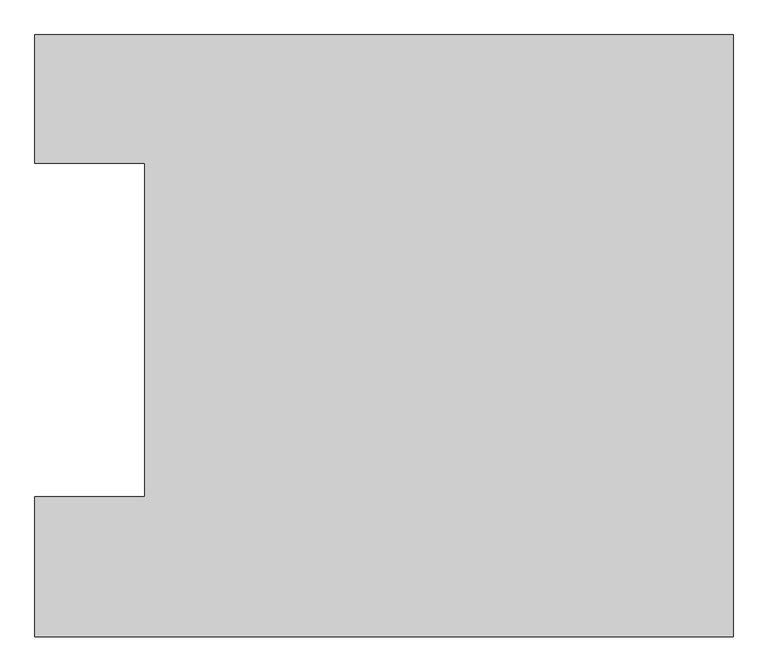
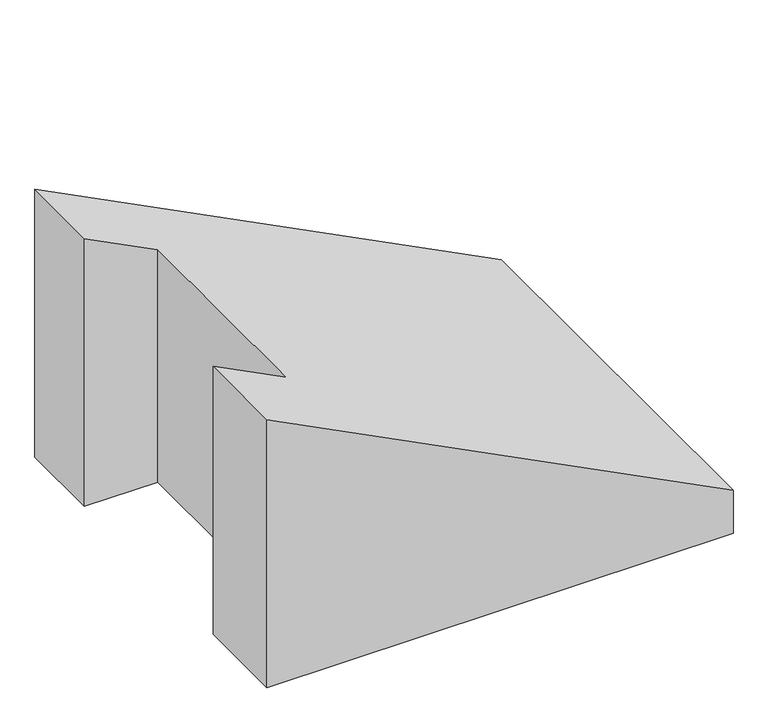
"""IFC4 building model written with IfcOpenShell, lengths in millimetres: proxy geometry, 0_3d."""

from ifc_helpers import new_model, si_unit, origin, place, context, project, spatial, faceted_brep, source, transform, mapped, element, save


def generic_models_337892f4(model_context):
    return source(origin(), model_context, "Body", "Brep", [
        faceted_brep([(6520.0, 5620.0, 638.6196708), (0.0, 5620.0, 3960.7256015), (0.0, 4420.0, 3960.7256015), (1025.0, 4420.0, 3438.4620158), (1025.0, 1305.0, 3438.4620158), (0.0, 1305.0, 3960.7256015), (0.0, 0.0, 3960.7256015), (6520.0, 0.0, 638.6196708), (1025.0, 1305.0, 0.0), (0.0, 1305.0, 0.0), (1025.0, 4420.0, 0.0), (0.0, 4420.0, 0.0), (6520.0, 5620.0, 0.0), (0.0, 5620.0, 0.0), (6520.0, 0.0, 0.0), (0.0, 0.0, 0.0)], [[[0, 1, 2, 3, 4, 5, 6, 7]], [[5, 4, 8, 9]], [[4, 3, 10, 8]], [[3, 2, 11, 10]], [[1, 0, 12, 13]], [[0, 7, 14, 12]], [[7, 6, 15, 14]], [[9, 15, 6, 5]], [[13, 11, 2, 1]], [[11, 13, 12, 14, 15, 9, 8, 10]]]),
    ])


if __name__ == "__main__":
    model = new_model("IFC4")
    model_context = context("Model", 3, world=origin())
    ifc_project = project(units=[si_unit("LENGTHUNIT", "METRE", prefix="MILLI")], contexts=[model_context])
    site = spatial("IfcSite", under=ifc_project)
    building = spatial("IfcBuilding", under=site)
    placement = place(None, origin())
    generic_models_shape = generic_models_337892f4(model_context)
    element("IfcBuildingElementProxy", 1, Name="0_3d", ObjectType="0_3d", at=placement, inside=building, context=model_context, shape_type="MappedRepresentation", body=[
        mapped(generic_models_shape, transform((0.0, 0.0, 0.0), x_axis=(1.0, 0.0, 0.0), y_axis=(0.0, 1.0, 0.0), z_axis=(0.0, 0.0, 1.0))),
    ])
    save(model, "model.ifc")

# Revit data of these elements
# Element 1 (IfcBuildingElementProxy, "0_3d")
#   Materials on its faces: "*1"
# Materials
#   "*1": class "Unassigned", colour RGB 175 175 175, transparency 0
